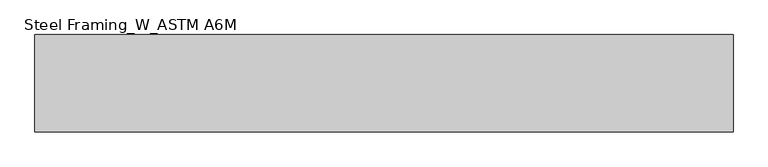
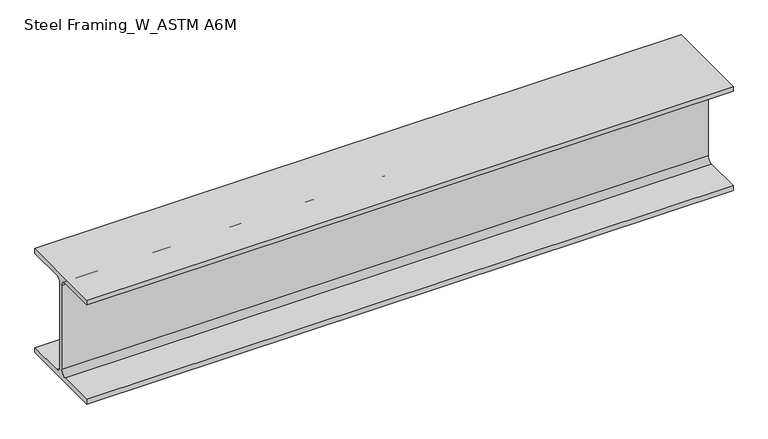
"""IFC4 building model written with IfcOpenShell, lengths in millimetres: beam geometry, Steel Framing_W_ASTM A6M : H_SB_AR_S02_W250x49.1_G5."""

import ifcopenshell
import ifcopenshell.guid

model = None  # the IFC model being written
_history = None  # IfcOwnerHistory: only IFC2X3 demands one
_inside = {}  # id of a spatial element -> (the spatial element, [elements in it])
_under = {}  # id of a project, library or spatial element -> (it, [spatial elements below it])
_declared = {}  # id of a project -> (the project, [libraries it declares])
_typed = {}  # id of a type object -> (the type object, [elements of that type])
_made_of = {}  # id of a material, layer set ... -> (it, [elements and type objects made of it])


def new_model(schema):
    """Start an empty IFC model of exactly this schema.

    Asked for "IFC4X3", IfcOpenShell would pick the latest addendum, in which some entities
    have other attributes; the version numbers below select the first issue.
    IFC2X3 requires an IfcOwnerHistory on every rooted entity: one is made here for all.
    """
    global model, _history
    if schema == "IFC4X3":
        model = ifcopenshell.file(schema_version=(4, 3, 0, 0))
    else:
        model = ifcopenshell.file(schema=schema)
    _inside.clear()
    _under.clear()
    _declared.clear()
    _typed.clear()
    _made_of.clear()
    _history = None
    if model.schema == "IFC2X3":
        org = make("IfcOrganization", Name="unknown")
        user = make(
            "IfcPersonAndOrganization",
            ThePerson=make("IfcPerson", FamilyName="unknown"),
            TheOrganization=org,
        )
        app = make(
            "IfcApplication",
            ApplicationDeveloper=org,
            Version="unknown",
            ApplicationFullName="unknown",
            ApplicationIdentifier="unknown",
        )
        _history = make(
            "IfcOwnerHistory",
            OwningUser=user,
            OwningApplication=app,
            ChangeAction="ADDED",
            CreationDate=0,
        )
    return model


def make(cls, **values):
    """One entity of the class cls with the attributes given. An attribute that is None is left unset."""
    return model.create_entity(
        cls, **{name: value for name, value in values.items() if value is not None}
    )


def rooted(cls, **values):
    """An entity with a GlobalId (a new one), such as an element, a storey or a relation."""
    return make(cls, GlobalId=ifcopenshell.guid.new(), OwnerHistory=_history, **values)


def si_unit(unit_type, name, prefix=None):
    """IfcSIUnit, for example si_unit("LENGTHUNIT", "METRE", prefix="MILLI")."""
    return make("IfcSIUnit", UnitType=unit_type, Prefix=prefix, Name=name)


def assignment(units):
    """IfcUnitAssignment: the units of a project."""
    return None if units is None else make("IfcUnitAssignment", Units=units)


def point(xyz):
    """IfcCartesianPoint."""
    return None if xyz is None else make("IfcCartesianPoint", Coordinates=xyz)


def direction(xyz):
    """IfcDirection."""
    return None if xyz is None else make("IfcDirection", DirectionRatios=xyz)


def frame(location, z_axis=None, x_axis=None):
    """IfcAxis2Placement3D, a coordinate frame: its origin and axes. An axis left out is left unset."""
    return make(
        "IfcAxis2Placement3D",
        Location=point(location),
        Axis=direction(z_axis),
        RefDirection=direction(x_axis),
    )


def frame_2d(location, x_axis=None):
    """IfcAxis2Placement2D, a coordinate frame in the plane: its origin and x axis."""
    return make(
        "IfcAxis2Placement2D", Location=point(location), RefDirection=direction(x_axis)
    )


def origin():
    """The frame at (0, 0, 0) with its axes left unset."""
    return frame((0.0, 0.0, 0.0))


def place(relative_to, where):
    """IfcLocalPlacement: puts the frame where relative to a parent placement (None: the world)."""
    return make(
        "IfcLocalPlacement", PlacementRelTo=relative_to, RelativePlacement=where
    )


def context(
    kind, dimensions, precision=None, world=None, true_north=None, identifier=None
):
    """IfcGeometricRepresentationContext, for example the 3D "Model" context."""
    return make(
        "IfcGeometricRepresentationContext",
        ContextIdentifier=identifier,
        ContextType=kind,
        CoordinateSpaceDimension=dimensions,
        Precision=precision,
        WorldCoordinateSystem=world,
        TrueNorth=true_north,
    )


def project(units=None, contexts=None):
    """IfcProject with its units and contexts."""
    return rooted(
        "IfcProject",
        Name="project",
        RepresentationContexts=contexts,
        UnitsInContext=assignment(units),
    )


def spatial(cls, under=None, at=None, **own):
    """A site, building, storey or space (cls), placed at a placement, below another one or the project."""
    s = rooted(cls, ObjectPlacement=at, **own)
    if under is not None:
        _under.setdefault(under.id(), (under, []))[1].append(s)
    return s


def polyline(points):
    """IfcPolyline through the points."""
    return make("IfcPolyline", Points=[point(p) for p in points])


def circle_curve(where, radius):
    """IfcCircle in the frame where."""
    return make("IfcCircle", Position=where, Radius=radius)


def trimmed(basis, trim1, trim2, sense, master):
    """IfcTrimmedCurve: the piece of a basis curve between two trims."""
    return make(
        "IfcTrimmedCurve",
        BasisCurve=basis,
        Trim1=trim1,
        Trim2=trim2,
        SenseAgreement=sense,
        MasterRepresentation=master,
    )


def segment(curve, same_sense, transition):
    """IfcCompositeCurveSegment."""
    return make(
        "IfcCompositeCurveSegment",
        Transition=transition,
        SameSense=same_sense,
        ParentCurve=curve,
    )


def composite_curve(segments, self_intersect=None):
    """IfcCompositeCurve: segments joined end to end."""
    return make("IfcCompositeCurve", Segments=segments, SelfIntersect=self_intersect)


def outline(outer, holes=None, kind="AREA"):
    """IfcArbitraryClosedProfileDef: a profile drawn as a closed curve; with holes, ...WithVoids."""
    if holes is None:
        return make("IfcArbitraryClosedProfileDef", ProfileType=kind, OuterCurve=outer)
    return make(
        "IfcArbitraryProfileDefWithVoids",
        ProfileType=kind,
        OuterCurve=outer,
        InnerCurves=holes,
    )


def extrude(swept, where, along, depth):
    """IfcExtrudedAreaSolid: the profile swept, set in the frame where, extruded along a direction by depth."""
    return make(
        "IfcExtrudedAreaSolid",
        SweptArea=swept,
        Position=where,
        ExtrudedDirection=direction(along),
        Depth=depth,
    )


def shape(context_of_items, identifier, shape_type, items):
    """IfcShapeRepresentation: the items that make up one representation, for example the "Body"."""
    return make(
        "IfcShapeRepresentation",
        ContextOfItems=context_of_items,
        RepresentationIdentifier=identifier,
        RepresentationType=shape_type,
        Items=items,
    )


def source(mapping_origin, context_of_items, identifier, shape_type, items):
    """IfcRepresentationMap: a shape defined once, which mapped items show again and again."""
    return make(
        "IfcRepresentationMap",
        MappingOrigin=mapping_origin,
        MappedRepresentation=shape(context_of_items, identifier, shape_type, items),
    )


def transform(
    local_origin,
    x_axis=None,
    y_axis=None,
    z_axis=None,
    scale=None,
    scale2=None,
    scale3=None,
    uniform=True,
):
    """IfcCartesianTransformationOperator3D, or its non-uniform kind. x_axis, y_axis, z_axis: its Axis1, 2, 3."""
    if uniform:
        return make(
            "IfcCartesianTransformationOperator3D",
            Axis1=direction(x_axis),
            Axis2=direction(y_axis),
            LocalOrigin=point(local_origin),
            Scale=scale,
            Axis3=direction(z_axis),
        )
    return make(
        "IfcCartesianTransformationOperator3DnonUniform",
        Axis1=direction(x_axis),
        Axis2=direction(y_axis),
        LocalOrigin=point(local_origin),
        Scale=scale,
        Axis3=direction(z_axis),
        Scale2=scale2,
        Scale3=scale3,
    )


def mapped(mapping_source, mapping_target):
    """IfcMappedItem: shows the shape of a source again, moved by a transform."""
    return make(
        "IfcMappedItem", MappingSource=mapping_source, MappingTarget=mapping_target
    )


def made_of(thing, what):
    """Note that an element or type object is made of a material, layer set ...; save() writes the relation."""
    if what is not None:
        _made_of.setdefault(what.id(), (what, []))[1].append(thing)
    return thing


def element(
    cls,
    number,
    at=None,
    inside=None,
    cuts=None,
    type_object=None,
    material=None,
    context=None,
    identifier="Body",
    shape_type=None,
    held_by="IfcProductDefinitionShape",
    body=None,
    shapes=None,
    **own,
):
    """One element of the class cls, such as IfcWall. Its Tag is "e" and its number.

    at: its placement. inside: the storey or other place that contains it. cuts: it is an
    opening in that element (IfcRelVoidsElement). A single representation is given by context,
    identifier, shape_type and body (its items); several are given by shapes. held_by: the class
    of the entity that holds the representations. save() writes the other relations.
    """
    e = rooted(cls, Tag="e%d" % number, ObjectPlacement=at, **own)
    if body is not None:
        shapes = [shape(context, identifier, shape_type, body)]
    if shapes is not None:
        e.Representation = make(held_by, Representations=shapes)
    if inside is not None:
        _inside.setdefault(inside.id(), (inside, []))[1].append(e)
    if cuts is not None:
        rooted(
            "IfcRelVoidsElement", RelatingBuildingElement=cuts, RelatedOpeningElement=e
        )
    if type_object is not None:
        _typed.setdefault(type_object.id(), (type_object, []))[1].append(e)
    return made_of(e, material)


def aggregate(whole, parts):
    """IfcRelAggregates: a whole, such as a stair, and the parts it consists of."""
    return rooted("IfcRelAggregates", RelatingObject=whole, RelatedObjects=parts)


def save(model, path):
    """Write the relations noted so far, then the file.

    IfcRelAggregates (storeys below a building ...), IfcRelContainedInSpatialStructure (elements
    in a storey), IfcRelDefinesByType, IfcRelAssociatesMaterial and IfcRelDeclares: one each for
    every whole, place, type object, material and project.
    """
    for whole, parts in _under.values():
        aggregate(whole, parts)
    for where, things in _inside.values():
        rooted(
            "IfcRelContainedInSpatialStructure",
            RelatedElements=things,
            RelatingStructure=where,
        )
    for kind, things in _typed.values():
        rooted("IfcRelDefinesByType", RelatedObjects=things, RelatingType=kind)
    for what, things in _made_of.values():
        rooted("IfcRelAssociatesMaterial", RelatedObjects=things, RelatingMaterial=what)
    for by, libraries in _declared.values():
        rooted("IfcRelDeclares", RelatingContext=by, RelatedDefinitions=libraries)
    model.write(path)


def steel_framing_w_astm_a6m_ee6b765e(model_context):
    return source(origin(), model_context, "Body", "SweptSolid", [
        extrude(outline(composite_curve([segment(polyline([(101.0, -112.5), (101.0, -123.5), (-101.0, -123.5), (-101.0, -112.5), (-16.385, -112.5)]), True, "CONTINUOUS"), segment(trimmed(circle_curve(frame_2d((-16.385, -99.8)), 12.7), [point((-16.385, -112.5))], [point((-3.685, -99.8))], True, "CARTESIAN"), True, "CONTINUOUS"), segment(polyline([(-3.685, -99.8), (-3.685, 99.8)]), True, "CONTINUOUS"), segment(trimmed(circle_curve(frame_2d((-16.385, 99.8)), 12.7), [point((-3.685, 99.8))], [point((-16.385, 112.5))], True, "CARTESIAN"), True, "CONTINUOUS"), segment(polyline([(-16.385, 112.5), (-101.0, 112.5), (-101.0, 123.5), (101.0, 123.5), (101.0, 112.5), (16.385, 112.5)]), True, "CONTINUOUS"), segment(trimmed(circle_curve(frame_2d((16.385, 99.8)), 12.7), [point((16.385, 112.5))], [point((3.685, 99.8))], True, "CARTESIAN"), True, "CONTINUOUS"), segment(polyline([(3.685, 99.8), (3.685, -99.8)]), True, "CONTINUOUS"), segment(trimmed(circle_curve(frame_2d((16.385, -99.8)), 12.7), [point((3.685, -99.8))], [point((16.385, -112.5))], True, "CARTESIAN"), True, "CONTINUOUS"), segment(polyline([(16.385, -112.5), (101.0, -112.5)]), True, "CONTINUOUS")], self_intersect=False)), frame((-634.3, 0.0, 0.0), z_axis=(1.0, 0.0, 0.0), x_axis=(0.0, 1.0, 0.0)), (0.0, 0.0, 1.0), 1451.3),
    ])


if __name__ == "__main__":
    model = new_model("IFC4")
    model_context = context("Model", 3, world=origin())
    ifc_project = project(units=[si_unit("LENGTHUNIT", "METRE", prefix="MILLI")], contexts=[model_context])
    site = spatial("IfcSite", under=ifc_project)
    building = spatial("IfcBuilding", under=site)
    placement = place(None, origin())
    steel_framing_w_astm_a6m_shape = steel_framing_w_astm_a6m_ee6b765e(model_context)
    element("IfcBeam", 1, ObjectType="Steel Framing_W_ASTM A6M : H_SB_AR_S02_W250x49.1_G5", at=placement, inside=building, context=model_context, shape_type="MappedRepresentation", body=[
        mapped(steel_framing_w_astm_a6m_shape, transform((0.0, 0.0, 0.0), x_axis=(1.0, 0.0, 0.0), y_axis=(0.0, 1.0, 0.0), z_axis=(0.0, 0.0, 1.0))),
    ])
    save(model, "model.ifc")

# Revit data of these elements
# Type "Steel Framing_W_ASTM A6M : H_SB_AR_S02_W250x49.1_G5"
#   Type Mark = "G5"
#   Section Name Key = "W10x33"
#   Width = 20.2 cm
#   Web Thickness = 0.737 cm
#   Web Fillet = 1.27 cm
#   Warping Constant = 212000.0 cm⁶
#   Torsional Moment of Inertia = 24.30 cm⁴
#   Section Area = 62.6 cm²
#   Plastic Modulus weak axis = 229.0 cm³
#   Plastic Modulus strong axis = 636.0 cm³
#   Perimeter = 1.27 m²/m
#   Nominal Weight = 49.10 kgf/m
#   Moment of Inertia weak axis = 1520.00 cm⁴
#   Moment of Inertia strong axis = 7120.00 cm⁴
#   Height = 24.7 cm
#   Flange Thickness = 1.1 cm
#   Elastic Modulus weak axis = 151.0 cm³
#   Elastic Modulus strong axis = 574.0 cm³
#   Centroid Vertical = 12.35 cm
#   Centroid Horizontal = 10.1 cm
#   Length [instance default] = 1500 mm
#   Structural Material [instance default] = Steel, 45-345
#   Bolt Spacing = 0
#   Assembly Code = ""
# Element 1 (IfcBeam, "Steel Framing_W_ASTM A6M : H_SB_AR_S02_W250x49.1_G5")
#   Materials on its faces: "Steel, 45-345"
# Materials
#   "Steel, 45-345": class "Metal", colour RGB 189 187 185, transparency 0, Description = "Steel 345 MPa", Cost = 0
